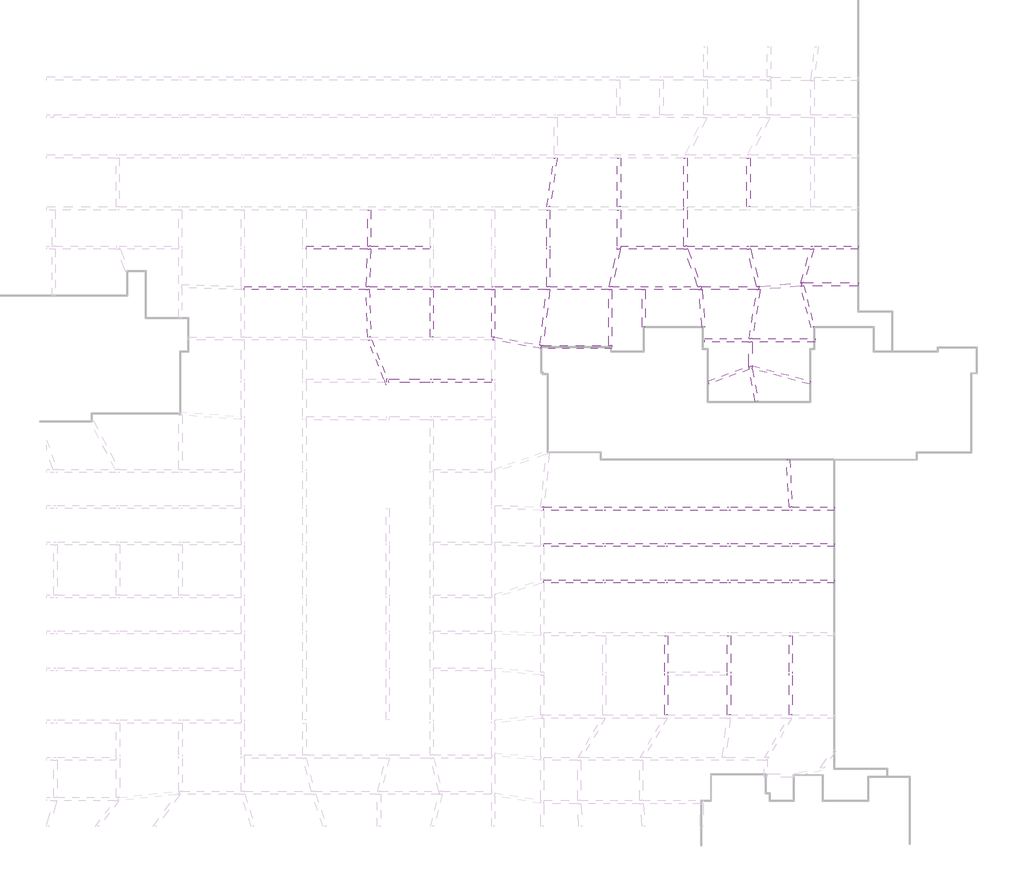
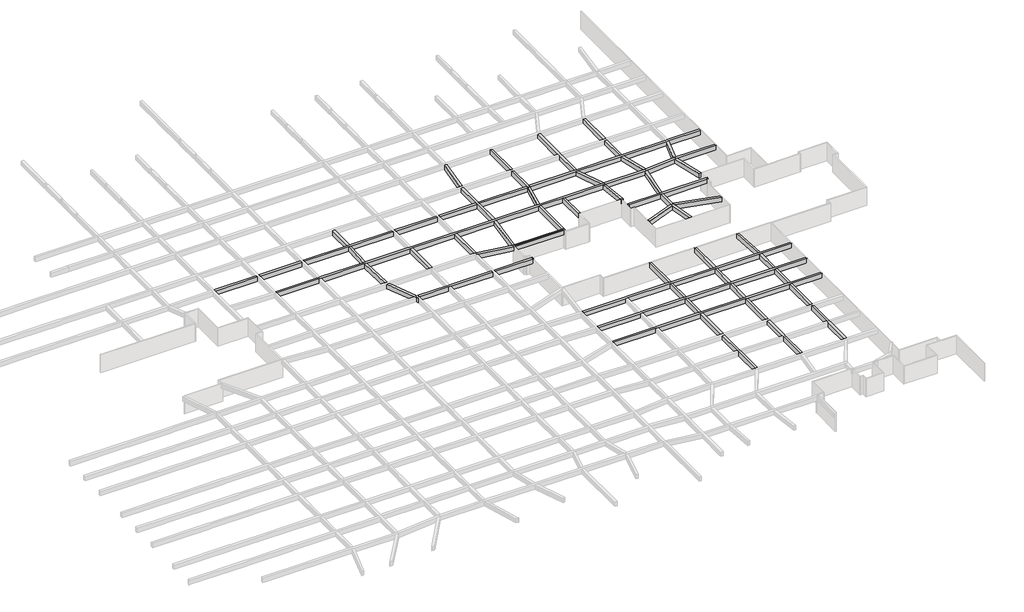
# One storey, part 43 of 45: 43 beams.
"""IFC4 building model written with IfcOpenShell, lengths in millimetres."""

from ifc_helpers import new_model, si_unit, frame, origin, place, context, project, spatial, polyline, outline, extrude, faceted_brep, element, save

model = new_model("IFC4")

# Units and contexts
model_context = context("Model", 3, world=origin())
ifc_project = project(units=[si_unit("LENGTHUNIT", "METRE", prefix="MILLI")], contexts=[model_context])

# Site, building, storey
site = spatial("IfcSite", under=ifc_project)
building = spatial("IfcBuilding", under=site)
storey = spatial("IfcBuildingStorey", under=building, Name="户型图", Elevation=0.0)

# Beams
placement = place(None, origin())
element("IfcBeam", 1, ObjectType="混凝土 - 矩形梁 : KL_beam", at=placement, inside=storey, context=model_context, shape_type="SweptSolid", body=[
    extrude(outline(polyline([(24974.8665178, 152479.7935386), (24570.9354888, 152479.7935386), (25428.027227, 158578.3181414), (25831.958256, 158578.3181414), (24974.8665178, 152479.7935386)])), frame((0.0, 0.0, 2500.0), z_axis=(0.0, 0.0, 1.0), x_axis=(1.0, 0.0, 0.0)), (0.0, 0.0, 1.0), 800.0),
])
element("IfcBeam", 2, ObjectType="混凝土 - 矩形梁 : KL_beam", at=placement, inside=storey, context=model_context, shape_type="Brep", body=[
    faceted_brep([(24944.7928364, 152079.7935386, 3300.0), (24544.7928364, 152079.7935386, 3300.0), (24544.7928364, 147579.5060773, 3300.0), (24544.7928364, 147179.5060773, 3300.0), (24544.7928364, 142504.5723204, 3300.0), (24944.7928364, 142504.5723204, 3300.0), (24944.7928364, 147179.5060773, 3300.0), (24944.7928364, 147579.5060773, 3300.0), (24544.7928364, 152079.7935386, 2500.0), (24544.7928364, 147579.5060773, 2500.0), (24544.7928364, 147179.5060773, 2500.0), (24544.7928364, 142504.5723204, 2500.0), (24944.7928364, 152079.7935386, 2500.0), (24944.7928364, 147579.5060773, 2500.0), (24944.7928364, 147179.5060773, 2500.0), (24944.7928364, 142504.5723204, 2500.0)], [[[0, 1, 2, 3, 4, 5, 6, 7]], [[1, 8, 9, 10, 11, 4, 3, 2]], [[8, 12, 13, 14, 15, 11, 10, 9]], [[12, 0, 7, 6, 5, 15, 14, 13]], [[1, 0, 12, 8]], [[5, 4, 11, 15]]]),
])
element("IfcBeam", 3, ObjectType="混凝土 - 矩形梁 : KL_beam", at=placement, inside=storey, context=model_context, shape_type="SweptSolid", body=[
    extrude(outline(polyline([(33758.170888, 152479.7935386), (33358.170888, 152479.7935386), (33358.170888, 158578.3181414), (33758.170888, 158578.3181414), (33758.170888, 152479.7935386)])), frame((0.0, 0.0, 2500.0), z_axis=(0.0, 0.0, 1.0), x_axis=(1.0, 0.0, 0.0)), (0.0, 0.0, 1.0), 800.0),
])
element("IfcBeam", 4, ObjectType="混凝土 - 矩形梁 : KL_beam", at=placement, inside=storey, context=model_context, shape_type="Brep", body=[
    faceted_brep([(42058.170888, 158578.3181414, 3300.0), (41658.170888, 158578.3181414, 3300.0), (41658.170888, 152479.7935386, 3300.0), (41658.170888, 152079.7935386, 3300.0), (41658.170888, 147579.7935386, 3300.0), (42058.170888, 147579.7935386, 3300.0), (42058.170888, 152079.7935386, 3300.0), (42058.170888, 152479.7935386, 3300.0), (41658.170888, 158578.3181414, 2500.0), (41658.170888, 152479.7935386, 2500.0), (41658.170888, 152079.7935386, 2500.0), (41658.170888, 147579.7935386, 2500.0), (42058.170888, 158578.3181414, 2500.0), (42058.170888, 152479.7935386, 2500.0), (42058.170888, 152079.7935386, 2500.0), (42058.170888, 147579.7935386, 2500.0)], [[[0, 1, 2, 3, 4, 5, 6, 7]], [[1, 8, 9, 10, 11, 4, 3, 2]], [[8, 12, 13, 14, 15, 11, 10, 9]], [[12, 0, 7, 6, 5, 15, 14, 13]], [[1, 0, 12, 8]], [[5, 4, 11, 15]]]),
])
element("IfcBeam", 5, ObjectType="混凝土 - 矩形梁 : KL_beam", at=placement, inside=storey, context=model_context, shape_type="Brep", body=[
    faceted_brep([(43849.7020076, 142104.5723204, 3300.0), (43849.7020076, 142504.5723204, 3300.0), (43423.9128831, 142504.5723204, 3300.0), (32726.4398492, 142504.5723204, 3300.0), (32317.5036113, 142504.5723204, 3300.0), (24944.7928364, 142504.5723204, 3300.0), (24544.7928364, 142504.5723204, 3300.0), (18058.170888, 142504.5723204, 3300.0), (17658.170888, 142504.5723204, 3300.0), (10373.3027926, 142504.5723204, 3300.0), (9973.3027926, 142504.5723204, 3300.0), (2402.7936694, 142504.5723204, 3300.0), (2002.5498517, 142504.5723204, 3300.0), (-5504.3123934, 142504.5723204, 3300.0), (-5904.3123934, 142504.5723204, 3300.0), (-13220.6748317, 142504.5723204, 3300.0), (-13220.6748317, 142104.5723204, 3300.0), (-5904.3123934, 142104.5723204, 3300.0), (-5504.3123934, 142104.5723204, 3300.0), (2001.2742725, 142104.5723204, 3300.0), (2401.4348111, 142104.5723204, 3300.0), (9973.3027926, 142104.5723204, 3300.0), (10373.3027926, 142104.5723204, 3300.0), (17658.170888, 142104.5723204, 3300.0), (18058.170888, 142104.5723204, 3300.0), (24519.4070452, 142104.5723204, 3300.0), (24922.2663133, 142104.5723204, 3300.0), (32279.492727, 142104.5723204, 3300.0), (32679.492727, 142104.5723204, 3300.0), (36462.5542012, 142104.5723204, 3300.0), (36862.5542012, 142104.5723204, 3300.0), (43526.283269, 142104.5723204, 3300.0), (43849.7020076, 142504.5723204, 2500.0), (43423.9128831, 142504.5723204, 2500.0), (32726.4398492, 142504.5723204, 2500.0), (32317.5036113, 142504.5723204, 2500.0), (24944.7928364, 142504.5723204, 2500.0), (24544.7928364, 142504.5723204, 2500.0), (18058.170888, 142504.5723204, 2500.0), (17658.170888, 142504.5723204, 2500.0), (10373.3027926, 142504.5723204, 2500.0), (9973.3027926, 142504.5723204, 2500.0), (2402.7936694, 142504.5723204, 2500.0), (2002.5498517, 142504.5723204, 2500.0), (-5504.3123934, 142504.5723204, 2500.0), (-5904.3123934, 142504.5723204, 2500.0), (-13220.6748317, 142504.5723204, 2500.0), (43849.7020076, 142104.5723204, 2500.0), (43526.283269, 142104.5723204, 2500.0), (36862.5542012, 142104.5723204, 2500.0), (36462.5542012, 142104.5723204, 2500.0), (32679.492727, 142104.5723204, 2500.0), (32279.492727, 142104.5723204, 2500.0), (24922.2663133, 142104.5723204, 2500.0), (24519.4070452, 142104.5723204, 2500.0), (18058.170888, 142104.5723204, 2500.0), (17658.170888, 142104.5723204, 2500.0), (10373.3027926, 142104.5723204, 2500.0), (9973.3027926, 142104.5723204, 2500.0), (2401.4348111, 142104.5723204, 2500.0), (2001.2742725, 142104.5723204, 2500.0), (-5504.3123934, 142104.5723204, 2500.0), (-5904.3123934, 142104.5723204, 2500.0), (-13220.6748317, 142104.5723204, 2500.0)], [[[0, 1, 2, 3, 4, 5, 6, 7, 8, 9, 10, 11, 12, 13, 14, 15, 16, 17, 18, 19, 20, 21, 22, 23, 24, 25, 26, 27, 28, 29, 30, 31]], [[1, 32, 33, 34, 35, 36, 37, 38, 39, 40, 41, 42, 43, 44, 45, 46, 15, 14, 13, 12, 11, 10, 9, 8, 7, 6, 5, 4, 3, 2]], [[32, 47, 48, 49, 50, 51, 52, 53, 54, 55, 56, 57, 58, 59, 60, 61, 62, 63, 46, 45, 44, 43, 42, 41, 40, 39, 38, 37, 36, 35, 34, 33]], [[47, 0, 31, 30, 29, 28, 27, 26, 25, 24, 23, 22, 21, 20, 19, 18, 17, 16, 63, 62, 61, 60, 59, 58, 57, 56, 55, 54, 53, 52, 51, 50, 49, 48]], [[16, 15, 46, 63]], [[0, 47, 32, 1]]]),
])
element("IfcBeam", 6, ObjectType="混凝土 - 矩形梁 : KL_beam", at=placement, inside=storey, context=model_context, shape_type="SweptSolid", body=[
    extrude(outline(polyline([(2402.7936694, 142504.5723204), (2002.5498517, 142504.5723204), (2165.8021358, 147179.5060773), (2566.0459535, 147179.5060773), (2402.7936694, 142504.5723204)])), frame((0.0, 0.0, 2500.0), z_axis=(0.0, 0.0, 1.0), x_axis=(1.0, 0.0, 0.0)), (0.0, 0.0, 1.0), 800.0),
])
element("IfcBeam", 7, ObjectType="混凝土 - 矩形梁 : KL_beam", at=placement, inside=storey, context=model_context, shape_type="SweptSolid", body=[
    extrude(outline(polyline([(2173.6750398, 152079.7935386), (2573.6750398, 152079.7935386), (2573.6750398, 147579.5060773), (2173.6750398, 147579.5060773), (2173.6750398, 152079.7935386)])), frame((0.0, 0.0, 2500.0), z_axis=(0.0, 0.0, 1.0), x_axis=(1.0, 0.0, 0.0)), (0.0, 0.0, 1.0), 800.0),
])
element("IfcBeam", 8, ObjectType="混凝土 - 矩形梁 : KL_beam", at=placement, inside=storey, context=model_context, shape_type="SweptSolid", body=[
    extrude(outline(polyline([(49536.7318858, 158578.3181414), (49936.7318858, 158578.3181414), (49936.7318858, 152479.7935386), (49536.7318858, 152479.7935386), (49536.7318858, 158578.3181414)])), frame((0.0, 0.0, 2500.0), z_axis=(0.0, 0.0, 1.0), x_axis=(1.0, 0.0, 0.0)), (0.0, 0.0, 1.0), 800.0),
    extrude(outline(polyline([(49536.7318858, 152079.7935386), (49936.7318858, 152079.7935386), (49936.7318858, 147579.7935386), (49536.7318858, 147579.7935386), (49536.7318858, 152079.7935386)])), frame((0.0, 0.0, 2500.0), z_axis=(0.0, 0.0, 1.0), x_axis=(1.0, 0.0, 0.0)), (0.0, 0.0, 1.0), 800.0),
])
element("IfcBeam", 9, ObjectType="混凝土 - 矩形梁 : KL_beam", at=placement, inside=storey, context=model_context, shape_type="Brep", body=[
    faceted_brep([(33358.170888, 147179.7935386, 3300.0), (33758.170888, 147179.7935386, 3300.0), (33758.170888, 147579.7935386, 3300.0), (33758.170888, 152079.7935386, 3300.0), (33358.170888, 152079.7935386, 3300.0), (33358.170888, 147579.5060773, 3300.0), (33358.170888, 147179.7935386, 2500.0), (33358.170888, 152079.7935386, 2500.0), (33358.170888, 147579.5060773, 2500.0), (33758.170888, 147179.7935386, 2500.0), (33758.170888, 152079.7935386, 2500.0), (33758.170888, 147579.7935386, 2500.0)], [[[0, 1, 2, 3, 4, 5]], [[6, 0, 5, 4, 7, 8]], [[9, 6, 8, 7, 10, 11]], [[1, 9, 11, 10, 3, 2]], [[4, 3, 10, 7]], [[1, 0, 6, 9]]]),
])
element("IfcBeam", 10, ObjectType="混凝土 - 矩形梁 : KL_beam", at=placement, inside=storey, context=model_context, shape_type="Brep", body=[
    faceted_brep([(63459.3246158, 147579.7935386, 3300.0), (63459.3246158, 147179.7935386, 3300.0), (63459.3246158, 147179.7935386, 2500.0), (63459.3246158, 147579.7935386, 2500.0), (57931.1254195, 147579.7935386, 3300.0), (57531.1254195, 147579.7935386, 3300.0), (49936.7318858, 147579.7935386, 3300.0), (49536.7318858, 147579.7935386, 3300.0), (42058.170888, 147579.7935386, 3300.0), (41658.170888, 147579.7935386, 3300.0), (33758.170888, 147579.7935386, 3300.0), (33758.170888, 147179.7935386, 3300.0), (41718.2427196, 147179.7935386, 3300.0), (42144.0318441, 147179.7935386, 3300.0), (49580.699658, 147179.7935386, 3300.0), (49993.0891817, 147179.7935386, 3300.0), (57464.435364, 147179.7935386, 3300.0), (57881.0788222, 147179.7935386, 3300.0), (33758.170888, 147179.7935386, 2500.0), (41718.2427196, 147179.7935386, 2500.0), (42144.0318441, 147179.7935386, 2500.0), (49580.699658, 147179.7935386, 2500.0), (49993.0891817, 147179.7935386, 2500.0), (57464.435364, 147179.7935386, 2500.0), (57881.0788222, 147179.7935386, 2500.0), (33758.170888, 147579.7935386, 2500.0), (41658.170888, 147579.7935386, 2500.0), (42058.170888, 147579.7935386, 2500.0), (49536.7318858, 147579.7935386, 2500.0), (49936.7318858, 147579.7935386, 2500.0), (57531.1254195, 147579.7935386, 2500.0), (57931.1254195, 147579.7935386, 2500.0)], [[[0, 1, 2, 3]], [[1, 0, 4, 5, 6, 7, 8, 9, 10, 11, 12, 13, 14, 15, 16, 17]], [[2, 1, 17, 16, 15, 14, 13, 12, 11, 18, 19, 20, 21, 22, 23, 24]], [[3, 2, 24, 23, 22, 21, 20, 19, 18, 25, 26, 27, 28, 29, 30, 31]], [[0, 3, 31, 30, 29, 28, 27, 26, 25, 10, 9, 8, 7, 6, 5, 4]], [[11, 10, 25, 18]]]),
])
element("IfcBeam", 11, ObjectType="混凝土 - 矩形梁 : KL_beam", at=placement, inside=storey, context=model_context, shape_type="Brep", body=[
    faceted_brep([(-21020.6748317, 147579.5060773, 3300.0), (-21020.6748317, 147179.5060773, 3300.0), (-13620.6748317, 147179.5060773, 3300.0), (-13620.6748317, 147579.5060773, 3300.0), (-21020.6748317, 147179.5060773, 2500.0), (-13620.6748317, 147179.5060773, 2500.0), (-21020.6748317, 147579.5060773, 2500.0), (-13620.6748317, 147579.5060773, 2500.0)], [[[0, 1, 2, 3]], [[1, 4, 5, 2]], [[4, 6, 7, 5]], [[6, 0, 3, 7]], [[1, 0, 6, 4]], [[3, 2, 5, 7]]]),
    faceted_brep([(33758.170888, 147179.5060773, 3300.0), (33758.170888, 147179.5060773, 2500.0), (33758.170888, 147179.7935386, 2500.0), (33758.170888, 147179.7935386, 3300.0), (33358.170888, 147179.7935386, 3300.0), (33358.170888, 147179.7935386, 2500.0), (33358.170888, 147579.5060773, 2500.0), (33358.170888, 147579.5060773, 3300.0), (24944.7928364, 147179.5060773, 3300.0), (24944.7928364, 147579.5060773, 3300.0), (24944.7928364, 147579.5060773, 2500.0), (24944.7928364, 147179.5060773, 2500.0), (33311.1914567, 147179.5060773, 3300.0), (33720.1276946, 147179.5060773, 3300.0), (33311.1914567, 147179.5060773, 2500.0), (33720.1276946, 147179.5060773, 2500.0)], [[[0, 1, 2, 3]], [[4, 5, 6, 7]], [[5, 4, 3, 2]], [[8, 9, 10, 11]], [[0, 3, 4, 7, 9, 8, 12, 13]], [[1, 0, 13, 12, 8, 11, 14, 15]], [[2, 1, 15, 14, 11, 10, 6, 5]], [[7, 6, 10, 9]]]),
    faceted_brep([(-13220.6748317, 147179.5060773, 3300.0), (-13220.6748317, 147579.5060773, 3300.0), (-13220.6748317, 147579.5060773, 2500.0), (-13220.6748317, 147179.5060773, 2500.0), (-5904.3123934, 147579.5060773, 3300.0), (-5904.3123934, 147179.5060773, 3300.0), (-5904.3123934, 147179.5060773, 2500.0), (-5904.3123934, 147579.5060773, 2500.0)], [[[0, 1, 2, 3]], [[4, 5, 6, 7]], [[1, 0, 5, 4]], [[0, 3, 6, 5]], [[3, 2, 7, 6]], [[2, 1, 4, 7]]]),
    faceted_brep([(-5504.3123934, 147579.5060773, 3300.0), (-5504.3123934, 147179.5060773, 3300.0), (2165.8021358, 147179.5060773, 3300.0), (2566.0459535, 147179.5060773, 3300.0), (9973.3027926, 147179.5060773, 3300.0), (9973.3027926, 147579.5060773, 3300.0), (2573.6750398, 147579.5060773, 3300.0), (2173.6750398, 147579.5060773, 3300.0), (-5504.3123934, 147179.5060773, 2500.0), (2165.8021358, 147179.5060773, 2500.0), (2566.0459535, 147179.5060773, 2500.0), (9973.3027926, 147179.5060773, 2500.0), (-5504.3123934, 147579.5060773, 2500.0), (2173.6750398, 147579.5060773, 2500.0), (2573.6750398, 147579.5060773, 2500.0), (9973.3027926, 147579.5060773, 2500.0)], [[[0, 1, 2, 3, 4, 5, 6, 7]], [[1, 8, 9, 10, 11, 4, 3, 2]], [[8, 12, 13, 14, 15, 11, 10, 9]], [[12, 0, 7, 6, 5, 15, 14, 13]], [[1, 0, 12, 8]], [[5, 4, 11, 15]]]),
    faceted_brep([(10373.3027926, 147179.5060773, 3300.0), (10373.3027926, 147579.5060773, 3300.0), (10373.3027926, 147579.5060773, 2500.0), (10373.3027926, 147179.5060773, 2500.0), (17658.170888, 147579.5060773, 3300.0), (17658.170888, 147179.5060773, 3300.0), (17658.170888, 147179.5060773, 2500.0), (17658.170888, 147579.5060773, 2500.0)], [[[0, 1, 2, 3]], [[4, 5, 6, 7]], [[1, 0, 5, 4]], [[0, 3, 6, 5]], [[3, 2, 7, 6]], [[2, 1, 4, 7]]]),
    faceted_brep([(18058.170888, 147579.5060773, 3300.0), (18058.170888, 147179.5060773, 3300.0), (24544.7928364, 147179.5060773, 3300.0), (24544.7928364, 147579.5060773, 3300.0), (18058.170888, 147179.5060773, 2500.0), (24544.7928364, 147179.5060773, 2500.0), (18058.170888, 147579.5060773, 2500.0), (24544.7928364, 147579.5060773, 2500.0)], [[[0, 1, 2, 3]], [[1, 4, 5, 2]], [[4, 6, 7, 5]], [[6, 0, 3, 7]], [[1, 0, 6, 4]], [[3, 2, 5, 7]]]),
])
element("IfcBeam", 12, ObjectType="混凝土 - 矩形梁 : KL_beam", at=placement, inside=storey, context=model_context, shape_type="SweptSolid", body=[
    extrude(outline(polyline([(32726.4398492, 142504.5723204), (32317.5036113, 142504.5723204), (33311.1914567, 147179.5060773), (33720.1276946, 147179.5060773), (32726.4398492, 142504.5723204)])), frame((0.0, 0.0, 2500.0), z_axis=(0.0, 0.0, 1.0), x_axis=(1.0, 0.0, 0.0)), (0.0, 0.0, 1.0), 800.0),
])
element("IfcBeam", 13, ObjectType="混凝土 - 矩形梁 : KL_beam", at=placement, inside=storey, context=model_context, shape_type="SweptSolid", body=[
    extrude(outline(polyline([(43849.7020076, 142504.5723204), (43423.9128831, 142504.5723204), (41718.2427196, 147179.7935386), (42144.0318441, 147179.7935386), (43849.7020076, 142504.5723204)])), frame((0.0, 0.0, 2500.0), z_axis=(0.0, 0.0, 1.0), x_axis=(1.0, 0.0, 0.0)), (0.0, 0.0, 1.0), 800.0),
])
element("IfcBeam", 14, ObjectType="混凝土 - 矩形梁 : KL_beam", at=placement, inside=storey, context=model_context, shape_type="Brep", body=[
    faceted_brep([(51018.2816924, 142104.5723204, 3300.0), (51000.8173152, 142504.5723204, 3300.0), (50753.3043756, 142504.5723204, 3300.0), (43849.7020076, 142504.5723204, 3300.0), (43849.7020076, 142104.5723204, 3300.0), (43927.811204, 142104.5723204, 3300.0), (50775.6048653, 142104.5723204, 3300.0), (51018.2816924, 142104.5723204, 2500.0), (43849.7020076, 142104.5723204, 2500.0), (43927.811204, 142104.5723204, 2500.0), (50775.6048653, 142104.5723204, 2500.0), (51000.8173152, 142504.5723204, 2500.0), (43849.7020076, 142504.5723204, 2500.0), (50753.3043756, 142504.5723204, 2500.0)], [[[0, 1, 2, 3, 4, 5, 6]], [[7, 0, 6, 5, 4, 8, 9, 10]], [[11, 7, 10, 9, 8, 12, 13]], [[1, 11, 13, 12, 3, 2]], [[4, 3, 12, 8]], [[1, 0, 7, 11]]]),
])
element("IfcBeam", 15, ObjectType="混凝土 - 矩形梁 : KL_beam", at=placement, inside=storey, context=model_context, shape_type="Brep", body=[
    faceted_brep([(56380.2686849, 142975.2133313, 3300.0), (56235.2737375, 142962.5279171, 3300.0), (51162.1536532, 142518.687421, 3300.0), (51000.8173152, 142504.5723204, 3300.0), (51018.2816924, 142104.5723204, 3300.0), (51182.8716123, 142118.9720726, 3300.0), (56236.5064832, 142561.1078334, 3300.0), (56397.733062, 142575.2133313, 3300.0), (51018.2816924, 142104.5723204, 2500.0), (51182.8716123, 142118.9720726, 2500.0), (56236.5064832, 142561.1078334, 2500.0), (56397.733062, 142575.2133313, 2500.0), (51000.8173152, 142504.5723204, 2500.0), (51162.1536532, 142518.687421, 2500.0), (56235.2737375, 142962.5279171, 2500.0), (56380.2686849, 142975.2133313, 2500.0)], [[[0, 1, 2, 3, 4, 5, 6, 7]], [[7, 6, 5, 4, 8, 9, 10, 11]], [[11, 10, 9, 8, 12, 13, 14, 15]], [[3, 2, 1, 0, 15, 14, 13, 12]], [[3, 12, 8, 4]], [[0, 7, 11, 15]]]),
])
element("IfcBeam", 16, ObjectType="混凝土 - 矩形梁 : KL_beam", at=placement, inside=storey, context=model_context, shape_type="Brep", body=[
    faceted_brep([(63459.2396085, 142975.2133313, 3300.0), (63459.2396085, 142575.2133313, 3300.0), (63459.2396085, 142575.2133313, 2500.0), (63459.2396085, 142975.2133313, 2500.0), (56655.6144787, 142975.2133313, 3300.0), (56380.2686849, 142975.2133313, 3300.0), (56397.733062, 142575.2133313, 3300.0), (56645.3581694, 142575.2133313, 3300.0), (56397.733062, 142575.2133313, 2500.0), (56645.3581694, 142575.2133313, 2500.0), (56380.2686849, 142975.2133313, 2500.0), (56655.6144787, 142975.2133313, 2500.0)], [[[0, 1, 2, 3]], [[1, 0, 4, 5, 6, 7]], [[2, 1, 7, 6, 8, 9]], [[3, 2, 9, 8, 10, 11]], [[0, 3, 11, 10, 5, 4]], [[5, 10, 8, 6]]]),
])
element("IfcBeam", 17, ObjectType="混凝土 - 矩形梁 : KL_beam", at=placement, inside=storey, context=model_context, shape_type="SweptSolid", body=[
    extrude(outline(polyline([(49580.699658, 147179.7935386), (49993.0891817, 147179.7935386), (51162.1536532, 142518.687421), (51000.8173152, 142504.5723204), (50753.3043756, 142504.5723204), (49580.699658, 147179.7935386)])), frame((0.0, 0.0, 2500.0), z_axis=(0.0, 0.0, 1.0), x_axis=(1.0, 0.0, 0.0)), (0.0, 0.0, 1.0), 800.0),
])
element("IfcBeam", 18, ObjectType="混凝土 - 矩形梁 : KL_beam", at=placement, inside=storey, context=model_context, shape_type="SweptSolid", body=[
    extrude(outline(polyline([(56380.2686849, 142975.2133313), (56235.2737375, 142962.5279171), (57464.435364, 147179.7935386), (57881.0788222, 147179.7935386), (56655.6144787, 142975.2133313), (56380.2686849, 142975.2133313)])), frame((0.0, 0.0, 2500.0), z_axis=(0.0, 0.0, 1.0), x_axis=(1.0, 0.0, 0.0)), (0.0, 0.0, 1.0), 800.0),
])
element("IfcBeam", 19, ObjectType="混凝土 - 矩形梁 : KL_beam", at=placement, inside=storey, context=model_context, shape_type="Brep", body=[
    faceted_brep([(23882.9959141, 135163.7066634, 3300.0), (23692.0574366, 135197.3742686, 3300.0), (18058.170888, 136190.7804734, 3300.0), (17875.6686207, 136222.9605472, 3300.0), (17840.6731553, 135822.9605472, 3300.0), (18058.0309094, 135784.6345106, 3300.0), (23848.0004486, 134763.7066634, 3300.0), (17840.6731553, 135822.9605472, 2500.0), (18058.0309094, 135784.6345106, 2500.0), (23848.0004486, 134763.7066634, 2500.0), (17875.6686207, 136222.9605472, 2500.0), (18058.170888, 136190.7804734, 2500.0), (23692.0574366, 135197.3742686, 2500.0), (23882.9959141, 135163.7066634, 2500.0)], [[[0, 1, 2, 3, 4, 5, 6]], [[6, 5, 4, 7, 8, 9]], [[9, 8, 7, 10, 11, 12, 13]], [[3, 2, 1, 0, 13, 12, 11, 10]], [[3, 10, 7, 4]], [[0, 6, 9, 13]]]),
])
element("IfcBeam", 20, ObjectType="混凝土 - 矩形梁 : KL_beam", at=placement, inside=storey, context=model_context, shape_type="Brep", body=[
    faceted_brep([(23882.9959141, 135163.7066634, 3300.0), (23848.0004486, 134763.7066634, 3300.0), (32679.492727, 134763.7066634, 3300.0), (32679.492727, 135163.7066634, 3300.0), (32279.492727, 135163.7066634, 3300.0), (24090.8839725, 135163.7066634, 3300.0), (23848.0004486, 134763.7066634, 2500.0), (32679.492727, 134763.7066634, 2500.0), (23882.9959141, 135163.7066634, 2500.0), (24090.8839725, 135163.7066634, 2500.0), (32279.492727, 135163.7066634, 2500.0), (32679.492727, 135163.7066634, 2500.0)], [[[0, 1, 2, 3, 4, 5]], [[1, 6, 7, 2]], [[6, 8, 9, 10, 11, 7]], [[8, 0, 5, 4, 3, 11, 10, 9]], [[0, 8, 6, 1]], [[3, 2, 7, 11]]]),
])
element("IfcBeam", 21, ObjectType="混凝土 - 矩形梁 : KL_beam", at=placement, inside=storey, context=model_context, shape_type="SweptSolid", body=[
    extrude(outline(polyline([(2001.2742725, 142104.5723204), (2401.4348111, 142104.5723204), (2568.0883739, 136222.9605472), (2167.9278354, 136222.9605472), (2001.2742725, 142104.5723204)])), frame((0.0, 0.0, 2500.0), z_axis=(0.0, 0.0, 1.0), x_axis=(1.0, 0.0, 0.0)), (0.0, 0.0, 1.0), 800.0),
])
element("IfcBeam", 22, ObjectType="混凝土 - 矩形梁 : KL_beam", at=placement, inside=storey, context=model_context, shape_type="SweptSolid", body=[
    extrude(outline(polyline([(9973.3027926, 142104.5723204), (10373.3027926, 142104.5723204), (10373.3027926, 136222.9605472), (9973.3027926, 136222.9605472), (9973.3027926, 142104.5723204)])), frame((0.0, 0.0, 2500.0), z_axis=(0.0, 0.0, 1.0), x_axis=(1.0, 0.0, 0.0)), (0.0, 0.0, 1.0), 800.0),
])
element("IfcBeam", 23, ObjectType="混凝土 - 矩形梁 : KL_beam", at=placement, inside=storey, context=model_context, shape_type="SweptSolid", body=[
    extrude(outline(polyline([(17875.6686207, 136222.9605472), (17658.170888, 136222.9605472), (17658.170888, 142104.5723204), (18058.170888, 142104.5723204), (18058.170888, 136190.7804734), (17875.6686207, 136222.9605472)])), frame((0.0, 0.0, 2500.0), z_axis=(0.0, 0.0, 1.0), x_axis=(1.0, 0.0, 0.0)), (0.0, 0.0, 1.0), 800.0),
])
element("IfcBeam", 24, ObjectType="混凝土 - 矩形梁 : KL_beam", at=placement, inside=storey, context=model_context, shape_type="SweptSolid", body=[
    extrude(outline(polyline([(23882.9959141, 135163.7066634), (23692.0574366, 135197.3742686), (24519.4070452, 142104.5723204), (24922.2663133, 142104.5723204), (24090.8839725, 135163.7066634), (23882.9959141, 135163.7066634)])), frame((0.0, 0.0, 2500.0), z_axis=(0.0, 0.0, 1.0), x_axis=(1.0, 0.0, 0.0)), (0.0, 0.0, 1.0), 800.0),
])
element("IfcBeam", 25, ObjectType="混凝土 - 矩形梁 : KL_beam", at=placement, inside=storey, context=model_context, shape_type="SweptSolid", body=[
    extrude(outline(polyline([(32679.492727, 135163.7066634), (32279.492727, 135163.7066634), (32279.492727, 142104.5723204), (32679.492727, 142104.5723204), (32679.492727, 135163.7066634)])), frame((0.0, 0.0, 2500.0), z_axis=(0.0, 0.0, 1.0), x_axis=(1.0, 0.0, 0.0)), (0.0, 0.0, 1.0), 800.0),
])
element("IfcBeam", 26, ObjectType="混凝土 - 矩形梁 : KL_beam", at=placement, inside=storey, context=model_context, shape_type="Brep", body=[
    faceted_brep([(44335.8161993, 137441.0538847, 3300.0), (43937.33832, 137406.1915876, 3300.0), (43937.33832, 137406.1915876, 2500.0), (44335.8161993, 137441.0538847, 2500.0), (43927.811204, 142104.5723204, 3300.0), (43849.7020076, 142104.5723204, 3300.0), (43526.283269, 142104.5723204, 3300.0), (43526.283269, 142104.5723204, 2500.0), (43849.7020076, 142104.5723204, 2500.0), (43927.811204, 142104.5723204, 2500.0)], [[[0, 1, 2, 3]], [[1, 0, 4, 5, 6]], [[2, 1, 6, 7]], [[3, 2, 7, 8, 9]], [[0, 3, 9, 4]], [[7, 6, 5, 4, 9, 8]]]),
])
element("IfcBeam", 27, ObjectType="混凝土 - 矩形梁 : KL_beam", at=placement, inside=storey, context=model_context, shape_type="SweptSolid", body=[
    extrude(outline(polyline([(36862.5542012, 137451.136222), (36462.5542012, 137451.136222), (36462.5542012, 142104.5723204), (36862.5542012, 142104.5723204), (36862.5542012, 137451.136222)])), frame((0.0, 0.0, 2500.0), z_axis=(0.0, 0.0, 1.0), x_axis=(1.0, 0.0, 0.0)), (0.0, 0.0, 1.0), 800.0),
])
element("IfcBeam", 28, ObjectType="混凝土 - 矩形梁 : KL_beam", at=placement, inside=storey, context=model_context, shape_type="Brep", body=[
    faceted_brep([(58079.2200875, 135993.2077532, 3300.0), (58079.2200875, 135593.2077532, 3300.0), (58079.2200875, 135593.2077532, 2500.0), (58079.2200875, 135993.2077532, 2500.0), (44279.2200875, 135993.2077532, 3300.0), (44279.2200875, 135993.2077532, 2500.0), (44279.2200875, 135593.2077532, 2500.0), (44279.2200875, 135593.2077532, 3300.0), (50212.645859, 135993.2077532, 3300.0), (49807.6598087, 135993.2077532, 3300.0), (49778.4759458, 135593.2077532, 3300.0), (50178.4759458, 135593.2077532, 3300.0), (49778.4759458, 135593.2077532, 2500.0), (50178.4759458, 135593.2077532, 2500.0), (49807.6598087, 135993.2077532, 2500.0), (50212.645859, 135993.2077532, 2500.0)], [[[0, 1, 2, 3]], [[4, 5, 6, 7]], [[1, 0, 8, 9, 4, 7, 10, 11]], [[2, 1, 11, 10, 7, 6, 12, 13]], [[3, 2, 13, 12, 6, 5, 14, 15]], [[0, 3, 15, 14, 5, 4, 9, 8]]]),
])
element("IfcBeam", 29, ObjectType="混凝土 - 矩形梁 : KL_beam", at=placement, inside=storey, context=model_context, shape_type="SweptSolid", body=[
    extrude(outline(polyline([(50212.645859, 135993.2077532), (49807.6598087, 135993.2077532), (50775.6048653, 142104.5723204), (51018.2816924, 142104.5723204), (51182.8716123, 142118.9720726), (50212.645859, 135993.2077532)])), frame((0.0, 0.0, 2500.0), z_axis=(0.0, 0.0, 1.0), x_axis=(1.0, 0.0, 0.0)), (0.0, 0.0, 1.0), 800.0),
])
element("IfcBeam", 30, ObjectType="混凝土 - 矩形梁 : KL_beam", at=placement, inside=storey, context=model_context, shape_type="Brep", body=[
    faceted_brep([(57925.0136781, 137473.1763903, 3300.0), (57537.0309802, 137375.8654139, 3300.0), (57537.0309802, 137375.8654139, 2500.0), (57925.0136781, 137473.1763903, 2500.0), (56645.3581694, 142575.2133313, 3300.0), (56539.0307264, 142575.2133313, 3300.0), (56397.733062, 142575.2133313, 3300.0), (56236.5064832, 142561.1078334, 3300.0), (56236.5064832, 142561.1078334, 2500.0), (56397.733062, 142575.2133313, 2500.0), (56539.0307264, 142575.2133313, 2500.0), (56645.3581694, 142575.2133313, 2500.0)], [[[0, 1, 2, 3]], [[1, 0, 4, 5, 6, 7]], [[2, 1, 7, 8]], [[3, 2, 8, 9, 10, 11]], [[0, 3, 11, 4]], [[7, 6, 9, 8]], [[4, 11, 10, 9, 6, 5]]]),
])
element("IfcBeam", 31, ObjectType="混凝土 - 矩形梁 : KL_beam", at=placement, inside=storey, context=model_context, shape_type="Brep", body=[
    faceted_brep([(49778.4759458, 132475.7100205, 3300.0), (50178.4759458, 132510.7054859, 3300.0), (50178.4759458, 132646.6731508, 3300.0), (50178.4759458, 135593.2077532, 3300.0), (49778.4759458, 135593.2077532, 3300.0), (49778.4759458, 132564.0495929, 3300.0), (49778.4759458, 132475.7100205, 2500.0), (49778.4759458, 135593.2077532, 2500.0), (49778.4759458, 132564.0495929, 2500.0), (50178.4759458, 132510.7054859, 2500.0), (50178.4759458, 135593.2077532, 2500.0), (50178.4759458, 132646.6731508, 2500.0)], [[[0, 1, 2, 3, 4, 5]], [[6, 0, 5, 4, 7, 8]], [[9, 6, 8, 7, 10, 11]], [[1, 9, 11, 10, 3, 2]], [[4, 3, 10, 7]], [[1, 0, 6, 9]]]),
])
element("IfcBeam", 32, ObjectType="混凝土 - 矩形梁 : KL_beam", at=placement, inside=storey, context=model_context, shape_type="Brep", body=[
    faceted_brep([(50939.4894781, 128194.7832755, 3300.0), (50545.5663769, 128125.3240044, 3300.0), (50545.5663769, 128125.3240044, 2500.0), (50939.4894781, 128194.7832755, 2500.0), (50229.9521044, 132218.7696835, 3300.0), (50178.4759458, 132510.7054859, 3300.0), (49778.4759458, 132475.7100205, 3300.0), (49834.381047, 132158.6564366, 3300.0), (49778.4759458, 132475.7100205, 2500.0), (49834.381047, 132158.6564366, 2500.0), (50178.4759458, 132510.7054859, 2500.0), (50229.9521044, 132218.7696835, 2500.0)], [[[0, 1, 2, 3]], [[1, 0, 4, 5, 6, 7]], [[2, 1, 7, 6, 8, 9]], [[3, 2, 9, 8, 10, 11]], [[0, 3, 11, 10, 5, 4]], [[5, 10, 8, 6]]]),
])
element("IfcBeam", 33, ObjectType="混凝土 - 矩形梁 : KL_beam", at=placement, inside=storey, context=model_context, shape_type="SweptSolid", body=[
    extrude(outline(polyline([(57467.8686173, 130693.4862712), (57364.3409992, 130307.1159407), (50229.9521044, 132218.7696835), (50178.4759458, 132510.7054859), (50178.4759458, 132646.6731508), (57467.8686173, 130693.4862712)])), frame((0.0, 0.0, 2500.0), z_axis=(0.0, 0.0, 1.0), x_axis=(1.0, 0.0, 0.0)), (0.0, 0.0, 1.0), 800.0),
])
element("IfcBeam", 34, ObjectType="混凝土 - 矩形梁 : KL_beam", at=placement, inside=storey, context=model_context, shape_type="SweptSolid", body=[
    extrude(outline(polyline([(44809.7929127, 130325.5260531), (44672.6989577, 130701.29892), (49778.4759458, 132564.0495929), (49778.4759458, 132475.7100205), (49834.381047, 132158.6564366), (44809.7929127, 130325.5260531)])), frame((0.0, 0.0, 2500.0), z_axis=(0.0, 0.0, 1.0), x_axis=(1.0, 0.0, 0.0)), (0.0, 0.0, 1.0), 800.0),
])
element("IfcBeam", 35, ObjectType="混凝土 - 矩形梁 : KL_beam", at=placement, inside=storey, context=model_context, shape_type="Brep", body=[
    faceted_brep([(24744.6709906, 130936.5288825, 3300.0), (24744.6709906, 130536.5288825, 3300.0), (24744.6709906, 130536.5288825, 2500.0), (24744.6709906, 130936.5288825, 2500.0), (18058.0309094, 130936.5288825, 3300.0), (18058.0309094, 130536.5288825, 3300.0), (18058.0309094, 130536.5288825, 2500.0), (18058.0309094, 130936.5288825, 2500.0)], [[[0, 1, 2, 3]], [[1, 0, 4, 5]], [[2, 1, 5, 6]], [[3, 2, 6, 7]], [[0, 3, 7, 4]], [[5, 4, 7, 6]]]),
    faceted_brep([(4809.3709906, 130936.5288825, 3300.0), (4809.3709906, 130936.5288825, 2500.0), (4809.3709906, 130536.5288825, 2500.0), (4809.3709906, 130536.5288825, 3300.0), (17658.0309094, 130936.5288825, 3300.0), (17658.0309094, 130536.5288825, 3300.0), (17658.0309094, 130536.5288825, 2500.0), (17658.0309094, 130936.5288825, 2500.0), (4900.9990644, 130536.5288825, 3300.0), (9973.3027926, 130536.5288825, 3300.0), (10373.3027926, 130536.5288825, 3300.0), (10373.3027926, 130936.5288825, 3300.0), (9973.3027926, 130936.5288825, 3300.0), (4900.9990644, 130536.5288825, 2500.0), (9973.3027926, 130536.5288825, 2500.0), (10373.3027926, 130536.5288825, 2500.0), (9973.3027926, 130936.5288825, 2500.0), (10373.3027926, 130936.5288825, 2500.0)], [[[0, 1, 2, 3]], [[4, 5, 6, 7]], [[0, 3, 8, 9, 10, 5, 4, 11, 12]], [[3, 2, 13, 14, 15, 6, 5, 10, 9, 8]], [[2, 1, 16, 17, 7, 6, 15, 14, 13]], [[1, 0, 12, 11, 4, 7, 17, 16]]]),
])
element("IfcBeam", 36, ObjectType="混凝土 - 矩形梁 : KL_beam", at=placement, inside=storey, context=model_context, shape_type="Brep", body=[
    faceted_brep([(2669.7438524, 135822.9605472, 3300.0), (2238.5848152, 135822.9605472, 3300.0), (4204.5051692, 130936.5288825, 3300.0), (4365.4340833, 130536.5288825, 3300.0), (4500.9990644, 130199.5727008, 3300.0), (4500.9990644, 130936.5288825, 3300.0), (4635.6642065, 130936.5288825, 3300.0), (2238.5848152, 135822.9605472, 2500.0), (4204.5051692, 130936.5288825, 2500.0), (4365.4340833, 130536.5288825, 2500.0), (4500.9990644, 130199.5727008, 2500.0), (2669.7438524, 135822.9605472, 2500.0), (4635.6642065, 130936.5288825, 2500.0), (4500.9990644, 130936.5288825, 2500.0)], [[[0, 1, 2, 3, 4, 5, 6]], [[1, 7, 8, 9, 10, 4, 3, 2]], [[7, 11, 12, 13, 10, 9, 8]], [[11, 0, 6, 12]], [[1, 0, 11, 7]], [[13, 5, 4, 10]], [[5, 13, 12, 6]]]),
])
element("IfcBeam", 37, ObjectType="混凝土 - 矩形梁 : KL_beam", at=placement, inside=storey, context=model_context, shape_type="Brep", body=[
    faceted_brep([(60459.4298456, 105882.8380814, 3300.0), (60459.4298456, 105482.8380814, 3300.0), (60459.4298456, 105482.8380814, 2500.0), (60459.4298456, 105882.8380814, 2500.0), (55199.4783436, 105882.8380814, 3300.0), (54799.4783436, 105882.8380814, 3300.0), (47494.6087163, 105882.8380814, 3300.0), (47094.6087163, 105882.8380814, 3300.0), (39666.3635798, 105882.8380814, 3300.0), (39266.3635798, 105882.8380814, 3300.0), (31925.9205959, 105882.8380814, 3300.0), (31525.9205959, 105882.8380814, 3300.0), (24178.3813476, 105882.8380814, 3300.0), (24178.3813476, 105534.4326096, 3300.0), (24178.3813476, 105482.8380814, 3300.0), (31525.9205959, 105482.8380814, 3300.0), (31925.9205959, 105482.8380814, 3300.0), (39266.3635798, 105482.8380814, 3300.0), (39666.3635798, 105482.8380814, 3300.0), (47094.6087163, 105482.8380814, 3300.0), (47494.6087163, 105482.8380814, 3300.0), (54799.4783436, 105482.8380814, 3300.0), (55199.4783436, 105482.8380814, 3300.0), (24178.3813476, 105482.8380814, 2500.0), (31525.9205959, 105482.8380814, 2500.0), (31925.9205959, 105482.8380814, 2500.0), (39266.3635798, 105482.8380814, 2500.0), (39666.3635798, 105482.8380814, 2500.0), (47094.6087163, 105482.8380814, 2500.0), (47494.6087163, 105482.8380814, 2500.0), (54799.4783436, 105482.8380814, 2500.0), (55199.4783436, 105482.8380814, 2500.0), (24178.3813476, 105534.4326096, 2500.0), (24178.3813476, 105882.8380814, 2500.0), (31525.9205959, 105882.8380814, 2500.0), (31925.9205959, 105882.8380814, 2500.0), (39266.3635798, 105882.8380814, 2500.0), (39666.3635798, 105882.8380814, 2500.0), (47094.6087163, 105882.8380814, 2500.0), (47494.6087163, 105882.8380814, 2500.0), (54799.4783436, 105882.8380814, 2500.0), (55199.4783436, 105882.8380814, 2500.0)], [[[0, 1, 2, 3]], [[1, 0, 4, 5, 6, 7, 8, 9, 10, 11, 12, 13, 14, 15, 16, 17, 18, 19, 20, 21, 22]], [[2, 1, 22, 21, 20, 19, 18, 17, 16, 15, 14, 23, 24, 25, 26, 27, 28, 29, 30, 31]], [[3, 2, 31, 30, 29, 28, 27, 26, 25, 24, 23, 32, 33, 34, 35, 36, 37, 38, 39, 40, 41]], [[0, 3, 41, 40, 39, 38, 37, 36, 35, 34, 33, 12, 11, 10, 9, 8, 7, 6, 5, 4]], [[12, 33, 32, 23, 14, 13]]]),
])
element("IfcBeam", 38, ObjectType="混凝土 - 矩形梁 : KL_beam", at=placement, inside=storey, context=model_context, shape_type="Brep", body=[
    faceted_brep([(60459.4298456, 110416.1887149, 3300.0), (60459.4298456, 110016.1887149, 3300.0), (60459.4298456, 110016.1887149, 2500.0), (60459.4298456, 110416.1887149, 2500.0), (55199.4783436, 110416.1887149, 3300.0), (54799.4783436, 110416.1887149, 3300.0), (47494.6087163, 110416.1887149, 3300.0), (47094.6087163, 110416.1887149, 3300.0), (39666.3635798, 110416.1887149, 3300.0), (39266.3635798, 110416.1887149, 3300.0), (31925.9205959, 110416.1887149, 3300.0), (31525.9205959, 110416.1887149, 3300.0), (24178.3813476, 110416.1887149, 3300.0), (24178.3813476, 110016.1887149, 3300.0), (31525.9205959, 110016.1887149, 3300.0), (31925.9205959, 110016.1887149, 3300.0), (39266.3635798, 110016.1887149, 3300.0), (39666.3635798, 110016.1887149, 3300.0), (47094.6087163, 110016.1887149, 3300.0), (47494.6087163, 110016.1887149, 3300.0), (54799.4783436, 110016.1887149, 3300.0), (55199.4783436, 110016.1887149, 3300.0), (24178.3813476, 110016.1887149, 2500.0), (31525.9205959, 110016.1887149, 2500.0), (31925.9205959, 110016.1887149, 2500.0), (39266.3635798, 110016.1887149, 2500.0), (39666.3635798, 110016.1887149, 2500.0), (47094.6087163, 110016.1887149, 2500.0), (47494.6087163, 110016.1887149, 2500.0), (54799.4783436, 110016.1887149, 2500.0), (55199.4783436, 110016.1887149, 2500.0), (24178.3813476, 110416.1887149, 2500.0), (31525.9205959, 110416.1887149, 2500.0), (31925.9205959, 110416.1887149, 2500.0), (39266.3635798, 110416.1887149, 2500.0), (39666.3635798, 110416.1887149, 2500.0), (47094.6087163, 110416.1887149, 2500.0), (47494.6087163, 110416.1887149, 2500.0), (54799.4783436, 110416.1887149, 2500.0), (55199.4783436, 110416.1887149, 2500.0)], [[[0, 1, 2, 3]], [[1, 0, 4, 5, 6, 7, 8, 9, 10, 11, 12, 13, 14, 15, 16, 17, 18, 19, 20, 21]], [[2, 1, 21, 20, 19, 18, 17, 16, 15, 14, 13, 22, 23, 24, 25, 26, 27, 28, 29, 30]], [[3, 2, 30, 29, 28, 27, 26, 25, 24, 23, 22, 31, 32, 33, 34, 35, 36, 37, 38, 39]], [[0, 3, 39, 38, 37, 36, 35, 34, 33, 32, 31, 12, 11, 10, 9, 8, 7, 6, 5, 4]], [[13, 12, 31, 22]]]),
])
element("IfcBeam", 39, ObjectType="混凝土 - 矩形梁 : KL_beam", at=placement, inside=storey, context=model_context, shape_type="Brep", body=[
    faceted_brep([(60459.4095922, 114958.1276627, 3300.0), (60459.4095922, 114558.1276627, 3300.0), (60459.4095922, 114558.1276627, 2500.0), (60459.4095922, 114958.1276627, 2500.0), (55189.2712569, 114958.1276627, 3300.0), (54788.7223185, 114958.1276627, 3300.0), (47494.6087163, 114958.1276627, 3300.0), (47094.6087163, 114958.1276627, 3300.0), (39666.3635798, 114958.1276627, 3300.0), (39266.3635798, 114958.1276627, 3300.0), (24198.8677371, 114958.1276627, 3300.0), (23981.8318538, 114958.1276627, 3300.0), (24178.3813476, 114951.2640031, 3300.0), (24178.3813476, 114558.1276627, 3300.0), (31525.9205959, 114558.1276627, 3300.0), (31925.9205959, 114558.1276627, 3300.0), (39266.3635798, 114558.1276627, 3300.0), (39666.3635798, 114558.1276627, 3300.0), (47094.6087163, 114558.1276627, 3300.0), (47494.6087163, 114558.1276627, 3300.0), (54799.4783436, 114558.1276627, 3300.0), (55199.4783436, 114558.1276627, 3300.0), (24178.3813476, 114558.1276627, 2500.0), (31525.9205959, 114558.1276627, 2500.0), (31925.9205959, 114558.1276627, 2500.0), (39266.3635798, 114558.1276627, 2500.0), (39666.3635798, 114558.1276627, 2500.0), (47094.6087163, 114558.1276627, 2500.0), (47494.6087163, 114558.1276627, 2500.0), (54799.4783436, 114558.1276627, 2500.0), (55199.4783436, 114558.1276627, 2500.0), (24178.3813476, 114951.2640031, 2500.0), (23981.8318538, 114958.1276627, 2500.0), (24198.8677371, 114958.1276627, 2500.0), (39266.3635798, 114958.1276627, 2500.0), (39666.3635798, 114958.1276627, 2500.0), (47094.6087163, 114958.1276627, 2500.0), (47494.6087163, 114958.1276627, 2500.0), (54788.7223185, 114958.1276627, 2500.0), (55189.2712569, 114958.1276627, 2500.0)], [[[0, 1, 2, 3]], [[1, 0, 4, 5, 6, 7, 8, 9, 10, 11, 12, 13, 14, 15, 16, 17, 18, 19, 20, 21]], [[2, 1, 21, 20, 19, 18, 17, 16, 15, 14, 13, 22, 23, 24, 25, 26, 27, 28, 29, 30]], [[3, 2, 30, 29, 28, 27, 26, 25, 24, 23, 22, 31, 32, 33, 34, 35, 36, 37, 38, 39]], [[0, 3, 39, 38, 37, 36, 35, 34, 33, 32, 11, 10, 9, 8, 7, 6, 5, 4]], [[31, 12, 11, 32]], [[12, 31, 22, 13]]]),
])
element("IfcBeam", 40, ObjectType="混凝土 - 矩形梁 : KL_beam", at=placement, inside=storey, context=model_context, shape_type="Brep", body=[
    faceted_brep([(39266.3635798, 120906.2363558, 3300.0), (39666.3635798, 120906.2363558, 3300.0), (39666.3635798, 120906.2363558, 2500.0), (39266.3635798, 120906.2363558, 2500.0), (39266.3635798, 114958.1276627, 3300.0), (39666.3635798, 114958.1276627, 3300.0), (39666.3635798, 114958.1276627, 2500.0), (39266.3635798, 114958.1276627, 2500.0)], [[[0, 1, 2, 3]], [[1, 0, 4, 5]], [[2, 1, 5, 6]], [[3, 2, 6, 7]], [[0, 3, 7, 4]], [[5, 4, 7, 6]]]),
    faceted_brep([(39266.3635798, 98874.9847154, 3300.0), (39666.3635798, 98874.9847154, 3300.0), (39666.3635798, 98874.9847154, 2500.0), (39266.3635798, 98874.9847154, 2500.0), (39266.3635798, 94353.2831144, 3300.0), (39266.3635798, 93953.2831144, 3300.0), (39266.3635798, 88990.7691713, 3300.0), (39666.3635798, 88990.7691713, 3300.0), (39666.3635798, 93953.2831144, 3300.0), (39666.3635798, 94353.2831144, 3300.0), (39666.3635798, 88990.7691713, 2500.0), (39666.3635798, 93953.2831144, 2500.0), (39666.3635798, 94353.2831144, 2500.0), (39266.3635798, 88990.7691713, 2500.0), (39266.3635798, 93953.2831144, 2500.0), (39266.3635798, 94353.2831144, 2500.0)], [[[0, 1, 2, 3]], [[1, 0, 4, 5, 6, 7, 8, 9]], [[2, 1, 9, 8, 7, 10, 11, 12]], [[3, 2, 12, 11, 10, 13, 14, 15]], [[0, 3, 15, 14, 13, 6, 5, 4]], [[7, 6, 13, 10]]]),
    faceted_brep([(39666.3635798, 99274.9847154, 3300.0), (39266.3635798, 99274.9847154, 3300.0), (39266.3635798, 99274.9847154, 2500.0), (39666.3635798, 99274.9847154, 2500.0), (39266.3635798, 105482.8380814, 3300.0), (39666.3635798, 105482.8380814, 3300.0), (39666.3635798, 105482.8380814, 2500.0), (39266.3635798, 105482.8380814, 2500.0)], [[[0, 1, 2, 3]], [[4, 5, 6, 7]], [[1, 0, 5, 4]], [[0, 3, 6, 5]], [[3, 2, 7, 6]], [[2, 1, 4, 7]]]),
    faceted_brep([(39666.3635798, 105882.8380814, 3300.0), (39266.3635798, 105882.8380814, 3300.0), (39266.3635798, 105882.8380814, 2500.0), (39666.3635798, 105882.8380814, 2500.0), (39266.3635798, 110016.1887149, 3300.0), (39666.3635798, 110016.1887149, 3300.0), (39666.3635798, 110016.1887149, 2500.0), (39266.3635798, 110016.1887149, 2500.0)], [[[0, 1, 2, 3]], [[4, 5, 6, 7]], [[1, 0, 5, 4]], [[0, 3, 6, 5]], [[3, 2, 7, 6]], [[2, 1, 4, 7]]]),
    faceted_brep([(39666.3635798, 110416.1887149, 3300.0), (39266.3635798, 110416.1887149, 3300.0), (39266.3635798, 110416.1887149, 2500.0), (39666.3635798, 110416.1887149, 2500.0), (39266.3635798, 114558.1276627, 3300.0), (39666.3635798, 114558.1276627, 3300.0), (39666.3635798, 114558.1276627, 2500.0), (39266.3635798, 114558.1276627, 2500.0)], [[[0, 1, 2, 3]], [[4, 5, 6, 7]], [[1, 0, 5, 4]], [[0, 3, 6, 5]], [[3, 2, 7, 6]], [[2, 1, 4, 7]]]),
])
element("IfcBeam", 41, ObjectType="混凝土 - 矩形梁 : KL_beam", at=placement, inside=storey, context=model_context, shape_type="Brep", body=[
    faceted_brep([(47094.6087163, 120906.2363558, 3300.0), (47494.6087163, 120906.2363558, 3300.0), (47494.6087163, 120906.2363558, 2500.0), (47094.6087163, 120906.2363558, 2500.0), (47094.6087163, 114958.1276627, 3300.0), (47494.6087163, 114958.1276627, 3300.0), (47494.6087163, 114958.1276627, 2500.0), (47094.6087163, 114958.1276627, 2500.0)], [[[0, 1, 2, 3]], [[1, 0, 4, 5]], [[2, 1, 5, 6]], [[3, 2, 6, 7]], [[0, 3, 7, 4]], [[5, 4, 7, 6]]]),
    faceted_brep([(47094.6087163, 98874.9847154, 3300.0), (47494.6087163, 98874.9847154, 3300.0), (47494.6087163, 98874.9847154, 2500.0), (47094.6087163, 98874.9847154, 2500.0), (47094.6087163, 94353.2831144, 3300.0), (47094.6087163, 93953.2831144, 3300.0), (47094.6087163, 88990.7691713, 3300.0), (47494.6087163, 88990.7691713, 3300.0), (47494.6087163, 93953.2831144, 3300.0), (47494.6087163, 94353.2831144, 3300.0), (47494.6087163, 88990.7691713, 2500.0), (47494.6087163, 93953.2831144, 2500.0), (47494.6087163, 94353.2831144, 2500.0), (47094.6087163, 88990.7691713, 2500.0), (47094.6087163, 93953.2831144, 2500.0), (47094.6087163, 94353.2831144, 2500.0)], [[[0, 1, 2, 3]], [[1, 0, 4, 5, 6, 7, 8, 9]], [[2, 1, 9, 8, 7, 10, 11, 12]], [[3, 2, 12, 11, 10, 13, 14, 15]], [[0, 3, 15, 14, 13, 6, 5, 4]], [[7, 6, 13, 10]]]),
    faceted_brep([(47494.6087163, 99274.9847154, 3300.0), (47094.6087163, 99274.9847154, 3300.0), (47094.6087163, 99274.9847154, 2500.0), (47494.6087163, 99274.9847154, 2500.0), (47094.6087163, 105482.8380814, 3300.0), (47494.6087163, 105482.8380814, 3300.0), (47494.6087163, 105482.8380814, 2500.0), (47094.6087163, 105482.8380814, 2500.0)], [[[0, 1, 2, 3]], [[4, 5, 6, 7]], [[1, 0, 5, 4]], [[0, 3, 6, 5]], [[3, 2, 7, 6]], [[2, 1, 4, 7]]]),
    faceted_brep([(47494.6087163, 105882.8380814, 3300.0), (47094.6087163, 105882.8380814, 3300.0), (47094.6087163, 105882.8380814, 2500.0), (47494.6087163, 105882.8380814, 2500.0), (47094.6087163, 110016.1887149, 3300.0), (47494.6087163, 110016.1887149, 3300.0), (47494.6087163, 110016.1887149, 2500.0), (47094.6087163, 110016.1887149, 2500.0)], [[[0, 1, 2, 3]], [[4, 5, 6, 7]], [[1, 0, 5, 4]], [[0, 3, 6, 5]], [[3, 2, 7, 6]], [[2, 1, 4, 7]]]),
    faceted_brep([(47494.6087163, 110416.1887149, 3300.0), (47094.6087163, 110416.1887149, 3300.0), (47094.6087163, 110416.1887149, 2500.0), (47494.6087163, 110416.1887149, 2500.0), (47094.6087163, 114558.1276627, 3300.0), (47494.6087163, 114558.1276627, 3300.0), (47494.6087163, 114558.1276627, 2500.0), (47094.6087163, 114558.1276627, 2500.0)], [[[0, 1, 2, 3]], [[4, 5, 6, 7]], [[1, 0, 5, 4]], [[0, 3, 6, 5]], [[3, 2, 7, 6]], [[2, 1, 4, 7]]]),
])
element("IfcBeam", 42, ObjectType="混凝土 - 矩形梁 : KL_beam", at=placement, inside=storey, context=model_context, shape_type="Brep", body=[
    faceted_brep([(55199.4783436, 114558.1276627, 3300.0), (54799.4783436, 114558.1276627, 3300.0), (54799.4783436, 110416.1887149, 3300.0), (55199.4783436, 110416.1887149, 3300.0), (54799.4783436, 114558.1276627, 2500.0), (54799.4783436, 110416.1887149, 2500.0), (55199.4783436, 114558.1276627, 2500.0), (55199.4783436, 110416.1887149, 2500.0)], [[[0, 1, 2, 3]], [[1, 4, 5, 2]], [[4, 6, 7, 5]], [[6, 0, 3, 7]], [[1, 0, 6, 4]], [[3, 2, 5, 7]]]),
    faceted_brep([(54799.4783436, 98874.9847154, 3300.0), (55199.4783436, 98874.9847154, 3300.0), (55199.4783436, 98874.9847154, 2500.0), (54799.4783436, 98874.9847154, 2500.0), (54799.4783436, 94353.2831144, 3300.0), (54799.4783436, 93953.2831144, 3300.0), (54799.4783436, 88990.7691713, 3300.0), (55199.4783436, 88990.7691713, 3300.0), (55199.4783436, 93953.2831144, 3300.0), (55199.4783436, 94353.2831144, 3300.0), (54799.4783436, 94353.2831144, 2500.0), (54799.4783436, 93953.2831144, 2500.0), (54799.4783436, 88990.7691713, 2500.0), (55199.4783436, 94353.2831144, 2500.0), (55199.4783436, 93953.2831144, 2500.0), (55199.4783436, 88990.7691713, 2500.0)], [[[0, 1, 2, 3]], [[1, 0, 4, 5, 6, 7, 8, 9]], [[0, 3, 10, 11, 12, 6, 5, 4]], [[3, 2, 13, 14, 15, 12, 11, 10]], [[2, 1, 9, 8, 7, 15, 14, 13]], [[7, 6, 12, 15]]]),
    faceted_brep([(55199.4783436, 99274.9847154, 3300.0), (54799.4783436, 99274.9847154, 3300.0), (54799.4783436, 99274.9847154, 2500.0), (55199.4783436, 99274.9847154, 2500.0), (54799.4783436, 105482.8380814, 3300.0), (55199.4783436, 105482.8380814, 3300.0), (55199.4783436, 105482.8380814, 2500.0), (54799.4783436, 105482.8380814, 2500.0)], [[[0, 1, 2, 3]], [[4, 5, 6, 7]], [[1, 0, 5, 4]], [[2, 1, 4, 7]], [[3, 2, 7, 6]], [[0, 3, 6, 5]]]),
    faceted_brep([(55199.4783436, 105882.8380814, 3300.0), (54799.4783436, 105882.8380814, 3300.0), (54799.4783436, 105882.8380814, 2500.0), (55199.4783436, 105882.8380814, 2500.0), (54799.4783436, 110016.1887149, 3300.0), (55199.4783436, 110016.1887149, 3300.0), (55199.4783436, 110016.1887149, 2500.0), (54799.4783436, 110016.1887149, 2500.0)], [[[0, 1, 2, 3]], [[4, 5, 6, 7]], [[1, 0, 5, 4]], [[2, 1, 4, 7]], [[3, 2, 7, 6]], [[0, 3, 6, 5]]]),
])
element("IfcBeam", 43, ObjectType="混凝土 - 矩形梁 : KL_beam", at=placement, inside=storey, context=model_context, shape_type="SweptSolid", body=[
    extrude(outline(polyline([(54477.5195916, 120896.229433), (54876.9714055, 120917.1638155), (55189.2712569, 114958.1276627), (54788.7223185, 114958.1276627), (54477.5195916, 120896.229433)])), frame((0.0, 0.0, 2500.0), z_axis=(0.0, 0.0, 1.0), x_axis=(1.0, 0.0, 0.0)), (0.0, 0.0, 1.0), 800.0),
])

save(model, "model.ifc")

# Revit data of these elements
# Type "混凝土 - 矩形梁 : KL_beam"
#   Length [instance default] = 1524 mm
#   b = 400 mm
#   h = 800 mm
#   Structural Material [instance default] = 混凝土 - 现场浇注混凝土
#   Assembly Code = ""
# Elements 1, 2, 3, 4, 5, 6, 7, 8, 9, 10, 11, 12, 13, 14, 15, 16, 17, 18, 19, 20, 21, 22, 23, 24, 25, 26, 27, 28, 29, 30, 31, 32, 33, 34, 35, 36, 37, 38, 39, 40, 41, 42, 43 (IfcBeam, "混凝土 - 矩形梁 : KL_beam")
#   Comments = ""
#   Structural Material = none
#   Phase Created = 新构造
# Materials
#   "混凝土 - 现场浇注混凝土": class "混凝土", colour RGB 192 192 192, transparency 0
